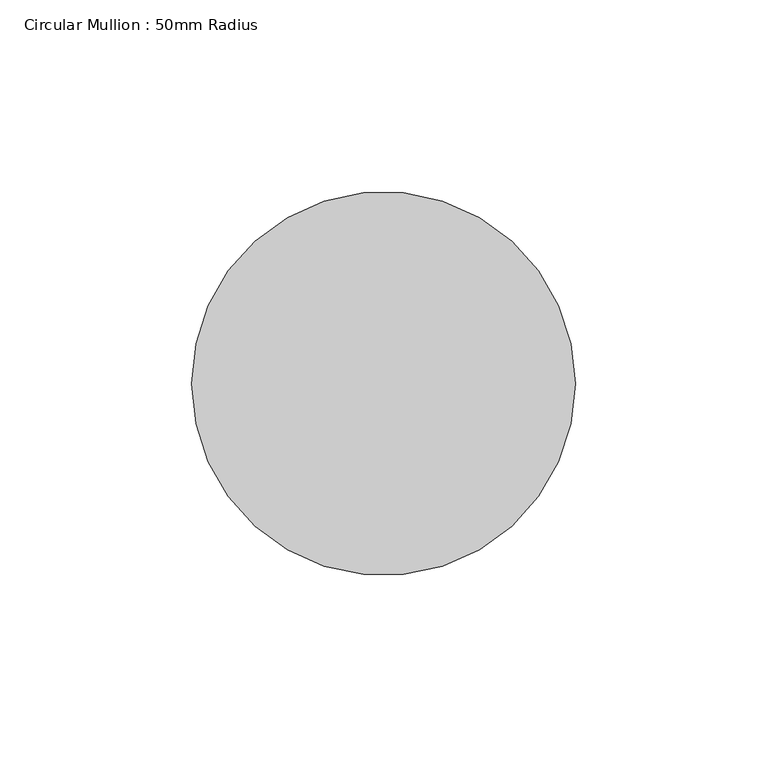
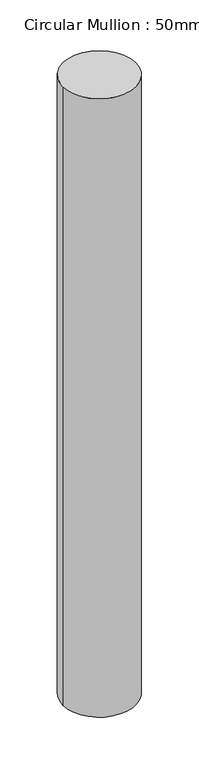
"""IFC4 building model written with IfcOpenShell, lengths in millimetres: member geometry, Circular Mullion : 50mm Radius."""

from ifc_helpers import new_model, si_unit, point, frame, origin, origin_2d, place, context, project, spatial, circle_curve, trimmed, segment, composite_curve, outline, extrude, source, transform, mapped, element, save


def circular_mullion_50mm_radius_64e291d9(model_context):
    return source(origin(), model_context, "Body", "SweptSolid", [
        extrude(outline(composite_curve([segment(trimmed(circle_curve(origin_2d(), 50.0), [point((50.0, 0.0))], [point((-50.0, 0.0))], False, "CARTESIAN"), True, "CONTINUOUS"), segment(trimmed(circle_curve(origin_2d(), 50.0), [point((-50.0, 0.0))], [point((50.0, 0.0))], False, "CARTESIAN"), True, "CONTINUOUS")], self_intersect=False)), frame((0.0, 0.0, -899.0975598), z_axis=(0.0, 0.0, 1.0), x_axis=(1.0, 0.0, 0.0)), (0.0, 0.0, 1.0), 899.0975598),
    ])


if __name__ == "__main__":
    model = new_model("IFC4")
    model_context = context("Model", 3, world=origin())
    ifc_project = project(units=[si_unit("LENGTHUNIT", "METRE", prefix="MILLI")], contexts=[model_context])
    site = spatial("IfcSite", under=ifc_project)
    building = spatial("IfcBuilding", under=site)
    placement = place(None, origin())
    circular_mullion_50mm_radius_shape = circular_mullion_50mm_radius_64e291d9(model_context)
    element("IfcMember", 1, ObjectType="Circular Mullion : 50mm Radius", at=placement, inside=building, context=model_context, shape_type="MappedRepresentation", body=[
        mapped(circular_mullion_50mm_radius_shape, transform((0.0, 0.0, 0.0), x_axis=(1.0, 0.0, 0.0), y_axis=(0.0, 1.0, 0.0), z_axis=(0.0, 0.0, 1.0))),
    ])
    save(model, "model.ifc")

# Revit data of these elements
# Type "Circular Mullion : 50mm Radius"
#   built-in parameter 1007350 = 0.164042 (stored number, unit not read)
# Element 1 (IfcMember, "Circular Mullion : 50mm Radius")
#   Materials on its faces: "Aluminium"
# Materials
#   "Aluminium": class "Metal", colour RGB 247 247 247, transparency 0, Description = "Aluminium 6061", Cost = 0
